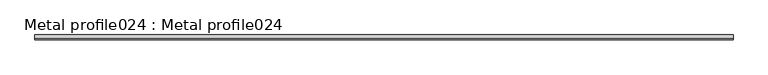
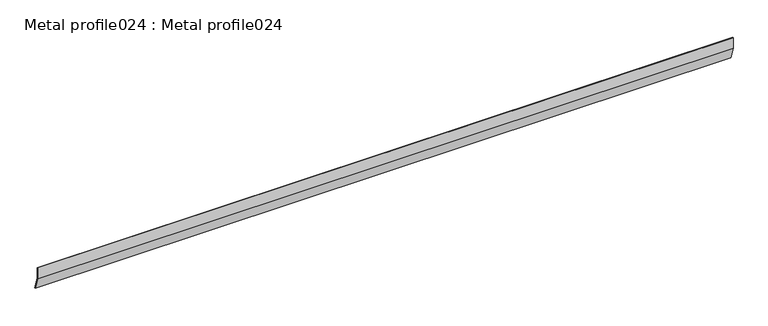
"""IFC4 building model written with IfcOpenShell, lengths in millimetres: proxy geometry, Metal profile024 : Metal profile024."""

from ifc_helpers import new_model, si_unit, frame, origin, place, context, project, spatial, polyline, outline, extrude, source, transform, mapped, element, save


def metal_profile024_metal_profile024_7d4e485c(model_context):
    return source(origin(), model_context, "Body", "SweptSolid", [
        extrude(outline(polyline([(10806.0039063, 43521.796875), (10806.0039063, 43554.671875), (10808.0039062, 43554.671875), (10808.0039062, 43522.112697), (10819.5960425, 43486.3233078), (10817.6933594, 43485.7070313), (10806.0039063, 43521.796875)])), frame((3694.2883192, 0.0, 0.0), z_axis=(1.0, 0.0, 0.0), x_axis=(0.0, 1.0, 0.0)), (0.0, 0.0, 1.0), 2000.0),
    ])


if __name__ == "__main__":
    model = new_model("IFC4")
    model_context = context("Model", 3, world=origin())
    ifc_project = project(units=[si_unit("LENGTHUNIT", "METRE", prefix="MILLI")], contexts=[model_context])
    site = spatial("IfcSite", under=ifc_project)
    building = spatial("IfcBuilding", under=site)
    placement = place(None, origin())
    metal_profile024_metal_profile024_shape = metal_profile024_metal_profile024_7d4e485c(model_context)
    element("IfcBuildingElementProxy", 1, Name="Metal profile024 : Metal profile024", ObjectType="Metal profile024 : Metal profile024", at=placement, inside=building, context=model_context, shape_type="MappedRepresentation", body=[
        mapped(metal_profile024_metal_profile024_shape, transform((0.0, 0.0, 0.0), x_axis=(1.0, 0.0, 0.0), y_axis=(0.0, 1.0, 0.0), z_axis=(0.0, 0.0, 1.0))),
    ])
    save(model, "model.ifc")

# Revit data of these elements
# Type "Metal profile024 : Metal profile024"
#   NameOverride = "Metal profile024"
# Element 1 (IfcBuildingElementProxy, "Metal profile024 : Metal profile024")
#   Materials on its faces: "ANGLE TRIM 3448"
# Materials
#   "ANGLE TRIM 3448": class "Unassigned", colour RGB 234 229 0, transparency 0
